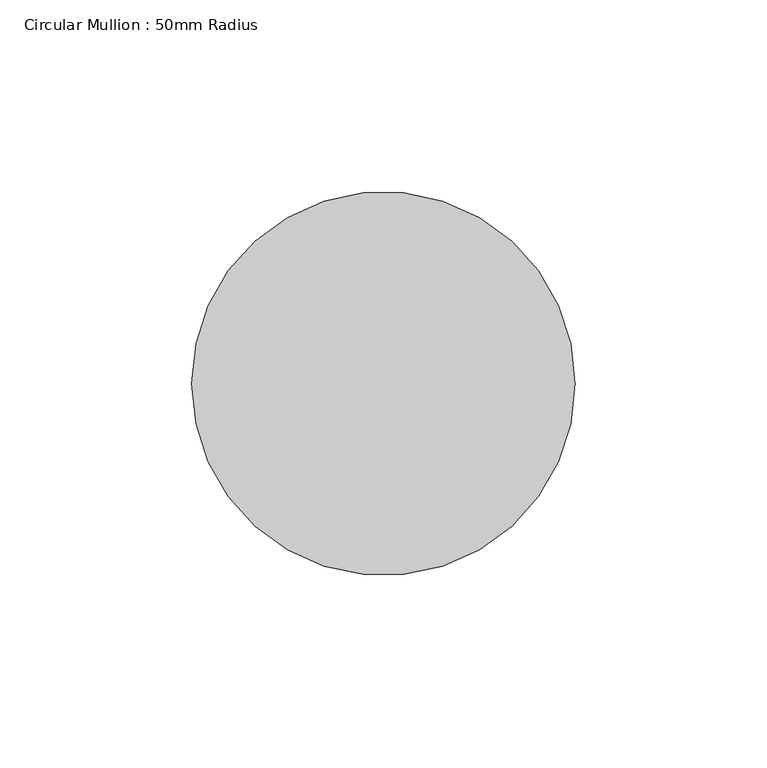
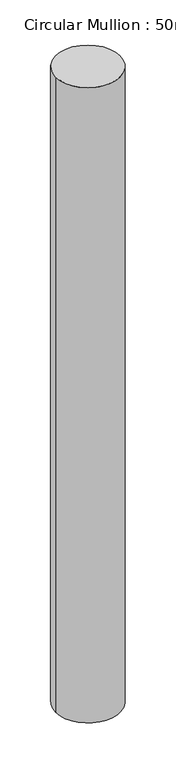
"""IFC4 building model written with IfcOpenShell, lengths in millimetres: member geometry, Circular Mullion : 50mm Radius."""

from ifc_helpers import new_model, si_unit, point, frame, origin, origin_2d, place, context, project, spatial, circle_curve, trimmed, segment, composite_curve, outline, extrude, source, transform, mapped, element, save


def circular_mullion_50mm_radius_b0b730fc(model_context):
    return source(origin(), model_context, "Body", "SweptSolid", [
        extrude(outline(composite_curve([segment(trimmed(circle_curve(origin_2d(), 50.0), [point((50.0, 0.0))], [point((-50.0, 0.0))], False, "CARTESIAN"), True, "CONTINUOUS"), segment(trimmed(circle_curve(origin_2d(), 50.0), [point((-50.0, 0.0))], [point((50.0, 0.0))], False, "CARTESIAN"), True, "CONTINUOUS")], self_intersect=False)), frame((0.0, 0.0, -1041.4650181), z_axis=(0.0, 0.0, 1.0), x_axis=(1.0, 0.0, 0.0)), (0.0, 0.0, 1.0), 1041.4650181),
    ])


if __name__ == "__main__":
    model = new_model("IFC4")
    model_context = context("Model", 3, world=origin())
    ifc_project = project(units=[si_unit("LENGTHUNIT", "METRE", prefix="MILLI")], contexts=[model_context])
    site = spatial("IfcSite", under=ifc_project)
    building = spatial("IfcBuilding", under=site)
    placement = place(None, origin())
    circular_mullion_50mm_radius_shape = circular_mullion_50mm_radius_b0b730fc(model_context)
    element("IfcMember", 1, ObjectType="Circular Mullion : 50mm Radius", at=placement, inside=building, context=model_context, shape_type="MappedRepresentation", body=[
        mapped(circular_mullion_50mm_radius_shape, transform((0.0, 0.0, 0.0), x_axis=(1.0, 0.0, 0.0), y_axis=(0.0, 1.0, 0.0), z_axis=(0.0, 0.0, 1.0))),
    ])
    save(model, "model.ifc")

# Revit data of these elements
# Type "Circular Mullion : 50mm Radius"
#   built-in parameter 1007350 = 0.164042 (stored number, unit not read)
# Element 1 (IfcMember, "Circular Mullion : 50mm Radius")
#   Materials on its faces: "Aluminium"
# Materials
#   "Aluminium": class "Metal", colour RGB 247 247 247, transparency 0, Description = "Aluminium 6061", Cost = 0
